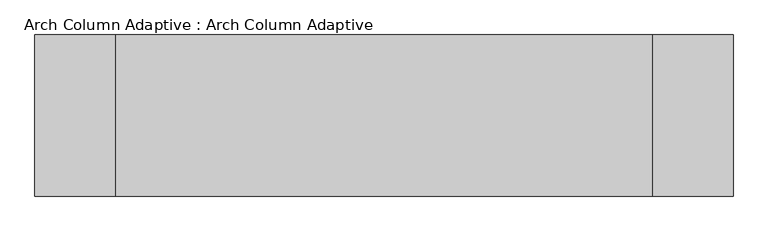
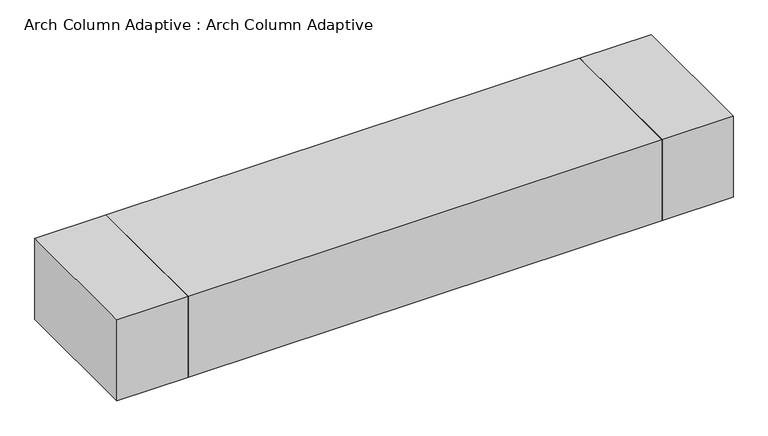
"""IFC4 building model written with IfcOpenShell, lengths in millimetres: proxy geometry, Arch Column Adaptive : Arch Column Adaptive."""

from ifc_helpers import new_model, si_unit, frame, origin, place, context, project, spatial, polyline, outline, extrude, source, transform, mapped, element, save


def arch_column_adaptive_arch_column_adaptive_7644014f(model_context):
    return source(origin(), model_context, "Body", "SweptSolid", [
        extrude(outline(polyline([(5000.0, -1500.0), (5000.0, 1500.0), (6500.0, 1500.0), (6500.0, -1500.0), (5000.0, -1500.0)])), frame((0.0, 0.0, 90038.8), z_axis=(0.0, 0.0, 1.0), x_axis=(1.0, 0.0, 0.0)), (0.0, 0.0, 1.0), 1800.0),
        extrude(outline(polyline([(-5000.0, 1500.0), (-5000.0, -1500.0), (-6500.0, -1500.0), (-6500.0, 1500.0), (-5000.0, 1500.0)])), frame((0.0, 0.0, 90038.8), z_axis=(0.0, 0.0, 1.0), x_axis=(1.0, 0.0, 0.0)), (0.0, 0.0, 1.0), 1800.0),
        extrude(outline(polyline([(-5000.0, -1500.0), (-5000.0, 1500.0), (5000.0, 1500.0), (5000.0, -1500.0), (-5000.0, -1500.0)])), frame((0.0, 0.0, 90038.8), z_axis=(0.0, 0.0, 1.0), x_axis=(1.0, 0.0, 0.0)), (0.0, 0.0, 1.0), 1800.0),
    ])


if __name__ == "__main__":
    model = new_model("IFC4")
    model_context = context("Model", 3, world=origin())
    ifc_project = project(units=[si_unit("LENGTHUNIT", "METRE", prefix="MILLI")], contexts=[model_context])
    site = spatial("IfcSite", under=ifc_project)
    building = spatial("IfcBuilding", under=site)
    placement = place(None, origin())
    arch_column_adaptive_arch_column_adaptive_shape = arch_column_adaptive_arch_column_adaptive_7644014f(model_context)
    element("IfcBuildingElementProxy", 1, Name="Arch Column Adaptive : Arch Column Adaptive", ObjectType="Arch Column Adaptive : Arch Column Adaptive", at=placement, inside=building, context=model_context, shape_type="MappedRepresentation", body=[
        mapped(arch_column_adaptive_arch_column_adaptive_shape, transform((0.0, 0.0, 0.0), x_axis=(1.0, 0.0, 0.0), y_axis=(0.0, 1.0, 0.0), z_axis=(0.0, 0.0, 1.0))),
    ])
    save(model, "model.ifc")

# Revit data of these elements
# Type "Arch Column Adaptive : Arch Column Adaptive"
#   Top Width = 3000 mm
#   Length [instance default] = 21000 mm
#   Height [instance default] = 50000 mm
#   Default Elevation = 0
# Element 1 (IfcBuildingElementProxy, "Arch Column Adaptive : Arch Column Adaptive")
#   Height = 90038.8 mm
